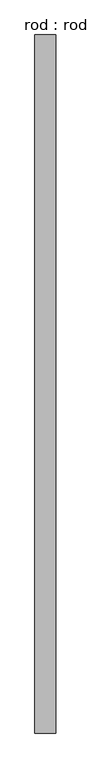
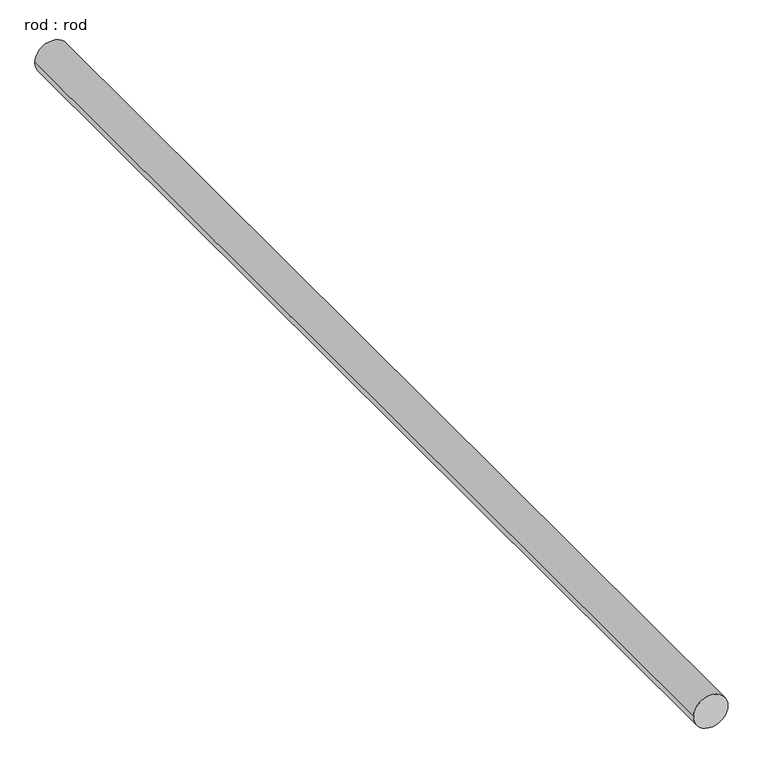
"""IFC4 building model written with IfcOpenShell, lengths in millimetres: proxy geometry, rod : rod."""

from ifc_helpers import new_model, si_unit, point, frame, frame_2d, origin, place, context, project, spatial, circle_curve, trimmed, segment, composite_curve, outline, extrude, source, transform, mapped, element, save


def rod_rod_481c27a9(model_context):
    return source(origin(), model_context, "Body", "SweptSolid", [
        extrude(outline(composite_curve([segment(trimmed(circle_curve(frame_2d((0.0108462, 0.0)), 200.0), [point((0.0108462, 200.0))], [point((0.0108462, -200.0))], False, "CARTESIAN"), True, "CONTINUOUS"), segment(trimmed(circle_curve(frame_2d((0.0108462, 0.0)), 200.0), [point((0.0108462, -200.0))], [point((0.0108462, 200.0))], False, "CARTESIAN"), True, "CONTINUOUS")], self_intersect=False)), frame((0.0, -2557.2713847, 0.0), z_axis=(0.0, 1.0, 0.0), x_axis=(0.0, 0.0, 1.0)), (0.0, 0.0, 1.0), 13300.0),
    ])


if __name__ == "__main__":
    model = new_model("IFC4")
    model_context = context("Model", 3, world=origin())
    ifc_project = project(units=[si_unit("LENGTHUNIT", "METRE", prefix="MILLI")], contexts=[model_context])
    site = spatial("IfcSite", under=ifc_project)
    building = spatial("IfcBuilding", under=site)
    placement = place(None, origin())
    rod_rod_shape = rod_rod_481c27a9(model_context)
    element("IfcBuildingElementProxy", 1, Name="rod : rod", ObjectType="rod : rod", at=placement, inside=building, context=model_context, shape_type="MappedRepresentation", body=[
        mapped(rod_rod_shape, transform((0.0, 0.0, 0.0), x_axis=(1.0, 0.0, 0.0), y_axis=(0.0, 1.0, 0.0), z_axis=(0.0, 0.0, 1.0))),
    ])
    save(model, "model.ifc")

# Revit data of these elements
# Type "rod : rod"
#   Default Elevation = 0
